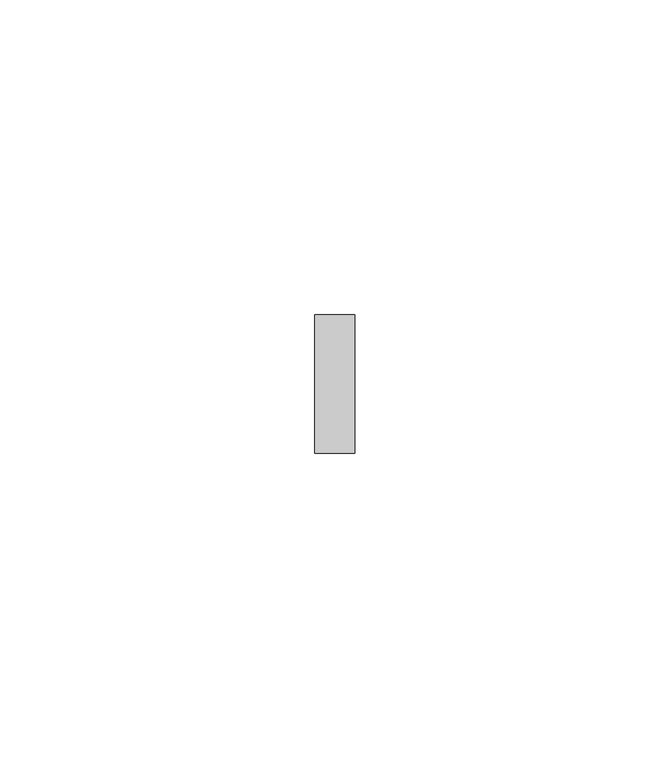
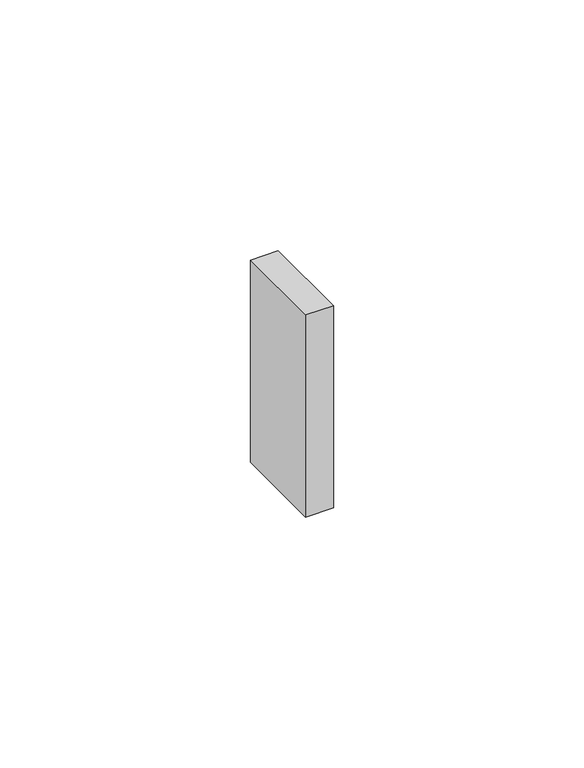
"""IFC4 building model written with IfcOpenShell, lengths in millimetres: proxy geometry, Panel:Panel:300402:Panel:300402 : Panel:Panel:300402:300124:Panel:300402:Panel:300402 : Panel:Panel:300402:300124 : Panel:Panel:300402:Panel:300402 : Panel:Panel:300402:300124:22 : Panel:Panel:300402:Panel:300402 : Panel:Panel:300402:300124:Panel:300402:Panel:300402 : Panel:Panel:300402:300124 : Panel:Panel:300402:Panel:300402 : Panel:Panel:300402:300124:300083."""

from ifc_helpers import new_model, si_unit, frame, origin, place, context, project, spatial, polyline, outline, extrude, source, transform, mapped, element, save


def generic_models_598ad444(model_context):
    return source(origin(), model_context, "Body", "SweptSolid", [
        extrude(outline(polyline([(560365.6617239, -578686.6186175), (560365.6617239, -578708.5652801), (560359.3117239, -578708.5652801), (560359.3117239, -578686.6186175), (560365.6617239, -578686.6186175)])), frame((0.0, 0.0, 6059.9247799), z_axis=(0.0, 0.0, 1.0), x_axis=(1.0, 0.0, 0.0)), (0.0, 0.0, 1.0), 49.2335472),
    ])


if __name__ == "__main__":
    model = new_model("IFC4")
    model_context = context("Model", 3, world=origin())
    ifc_project = project(units=[si_unit("LENGTHUNIT", "METRE", prefix="MILLI")], contexts=[model_context])
    site = spatial("IfcSite", under=ifc_project)
    building = spatial("IfcBuilding", under=site)
    placement = place(None, origin())
    generic_models_shape = generic_models_598ad444(model_context)
    element("IfcBuildingElementProxy", 1, Name="Panel:Panel:300402:Panel:300402 : Panel:Panel:300402:300124:Panel:300402:Panel:300402 : Panel:Panel:300402:300124 : Panel:Panel:300402:Panel:300402 : Panel:Panel:300402:300124:22 : Panel:Panel:300402:Panel:300402 : Panel:Panel:300402:300124:Panel:300402:Panel:300402 : Panel:Panel:300402:300124 : Panel:Panel:300402:Panel:300402 : Panel:Panel:300402:300124:300083", ObjectType="Panel:Panel:300402:Panel:300402 : Panel:Panel:300402:300124:Panel:300402:Panel:300402 : Panel:Panel:300402:300124 : Panel:Panel:300402:Panel:300402 : Panel:Panel:300402:300124:22 : Panel:Panel:300402:Panel:300402 : Panel:Panel:300402:300124:Panel:300402:Panel:300402 : Panel:Panel:300402:300124 : Panel:Panel:300402:Panel:300402 : Panel:Panel:300402:300124:300083", at=placement, inside=building, context=model_context, shape_type="MappedRepresentation", body=[
        mapped(generic_models_shape, transform((0.0, 0.0, 0.0), x_axis=(1.0, 0.0, 0.0), y_axis=(0.0, 1.0, 0.0), z_axis=(0.0, 0.0, 1.0))),
    ])
    save(model, "model.ifc")

# Revit data of these elements
# Type "Panel:Panel:300402:Panel:300402 : Panel:Panel:300402:300124:Panel:300402:Panel:300402 : Panel:Panel:300402:300124 : Panel:Panel:300402:Panel:300402 : Panel:Panel:300402:300124:22 : Panel:Panel:300402:Panel:300402 : Panel:Panel:300402:300124:Panel:300402:Panel:300402 : Panel:Panel:300402:300124 : Panel:Panel:300402:Panel:300402 : Panel:Panel:300402:300124:300083"
#   NameOverride = "Panel:Panel:300402:Panel:300402 : Panel:Panel:300402:300124:Panel:300402:Panel:300402 : Panel:Panel:300402:300124 : Panel:Panel:300402:Panel:300402 : Panel:Panel:300402:300124:300083"
#   ObjectTypeOverride = "Panel:300402:Panel:300402 : Panel:Panel:300402:300124 : Panel:Panel:300402:Panel:300402 : Panel:Panel:300402:300124"
#   Reference = "Panel"
#   Tag = "300083"
# Element 1 (IfcBuildingElementProxy, "Panel:Panel:300402:Panel:300402 : Panel:Panel:300402:300124:Panel:300402:Panel:300402 : Panel:Panel:300402:300124 : Panel:Panel:300402:Panel:300402 : Panel:Panel:300402:300124:22 : Panel:Panel:300402:Panel:300402 : Panel:Panel:300402:300124:Panel:300402:Panel:300402 : Panel:Panel:300402:300124 : Panel:Panel:300402:Panel:300402 : Panel:Panel:300402:300124:300083")
#   Materials on its faces: "1/4\" UV & WEATHER RESISTANT SPACER - FROM/BACK OF GIRT"
# Materials
#   "1/4\" UV & WEATHER RESISTANT SPACER - FROM/BACK OF GIRT": class "Unassigned", colour RGB 187 187 187, transparency 0, Keynote = "M07420000.01", Cost = 0
